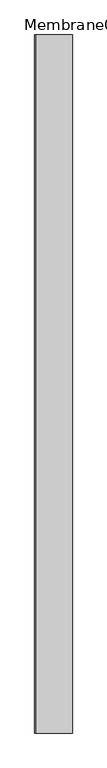
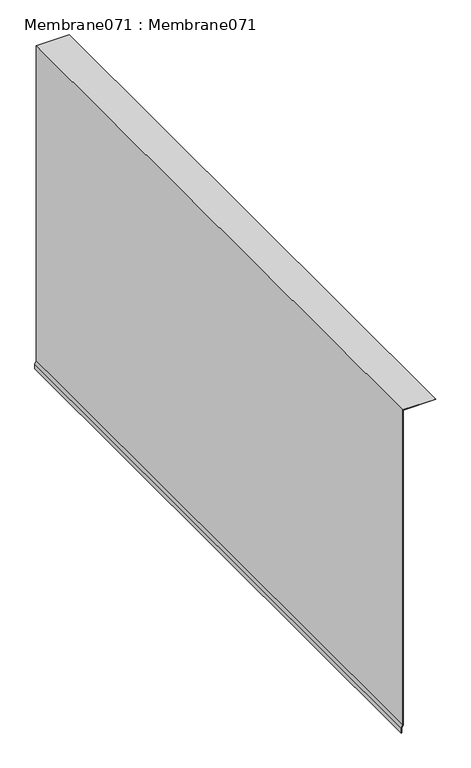
"""IFC4 building model written with IfcOpenShell, lengths in millimetres: proxy geometry, Membrane071 : Membrane071."""

from ifc_helpers import new_model, si_unit, frame, origin, place, context, project, spatial, polyline, outline, extrude, source, transform, mapped, element, save


def membrane071_membrane071_fd57ed91(model_context):
    return source(origin(), model_context, "Body", "SweptSolid", [
        extrude(outline(polyline([(36138.3085937, -8328.1069346), (36138.3085937, -8431.8487174), (35090.0493894, -8431.8487174), (35078.8241242, -8435.9343798), (35063.2418125, -8435.9343798), (35063.2418125, -8434.9343798), (35078.6477972, -8434.9343798), (35089.8730624, -8430.8487174), (36137.3085937, -8430.8487174), (36137.3085937, -8328.1069346), (36138.3085937, -8328.1069346)])), frame((0.0, 4540.4513244, 0.0), z_axis=(0.0, 1.0, 0.0), x_axis=(0.0, 0.0, 1.0)), (0.0, 0.0, 1.0), 2000.0),
    ])


if __name__ == "__main__":
    model = new_model("IFC4")
    model_context = context("Model", 3, world=origin())
    ifc_project = project(units=[si_unit("LENGTHUNIT", "METRE", prefix="MILLI")], contexts=[model_context])
    site = spatial("IfcSite", under=ifc_project)
    building = spatial("IfcBuilding", under=site)
    placement = place(None, origin())
    membrane071_membrane071_shape = membrane071_membrane071_fd57ed91(model_context)
    element("IfcBuildingElementProxy", 1, Name="Membrane071 : Membrane071", ObjectType="Membrane071 : Membrane071", at=placement, inside=building, context=model_context, shape_type="MappedRepresentation", body=[
        mapped(membrane071_membrane071_shape, transform((0.0, 0.0, 0.0), x_axis=(1.0, 0.0, 0.0), y_axis=(0.0, 1.0, 0.0), z_axis=(0.0, 0.0, 1.0))),
    ])
    save(model, "model.ifc")

# Revit data of these elements
# Type "Membrane071 : Membrane071"
#   NameOverride = "Membrane071"
# Element 1 (IfcBuildingElementProxy, "Membrane071 : Membrane071")
#   Materials on its faces: "(2) LAYERS OF ICE & WATER SHIELD (BITUTHANE) UNDER STUCCO"
# Materials
#   "(2) LAYERS OF ICE & WATER SHIELD (BITUTHANE) UNDER STUCCO": class "Unassigned", colour RGB 186 255 159, transparency 0, Cost = 0
